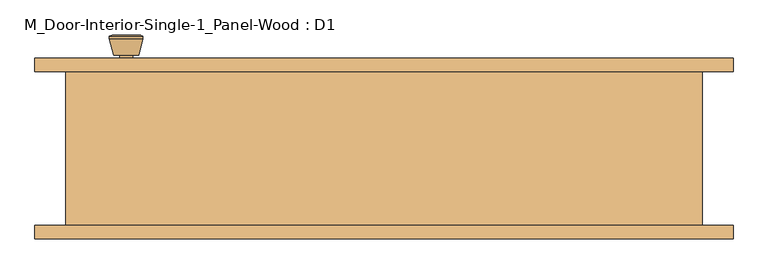
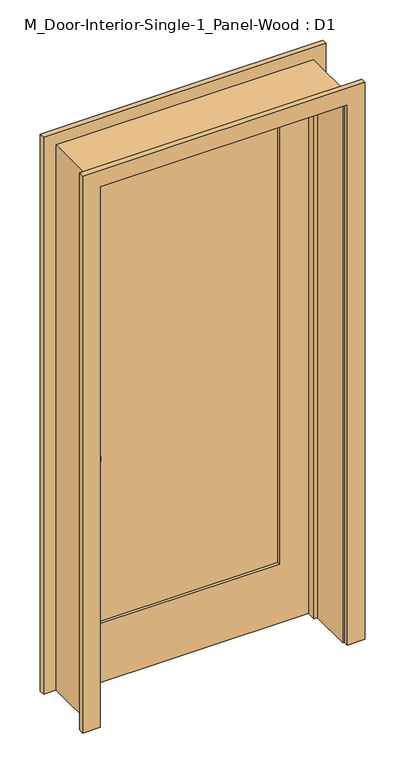
"""IFC4 building model written with IfcOpenShell, lengths in millimetres: door geometry, M_Door-Interior-Single-1_Panel-Wood : D1."""

from ifc_helpers import new_model, si_unit, point, frame, frame_2d, origin, place, context, project, spatial, polyline, circle_curve, trimmed, segment, composite_curve, outline, extrude, faceted_brep, source, transform, mapped, element, save
from ifc_brep_helpers import plane_surface, cylinder_surface, revolved_surface, advanced_brep


def m_door_interior_single_1_panel_wood_d1_706e19ec(model_context):
    return source(origin(), model_context, "Body", "SolidModel", [
        advanced_brep(
        [(-385.0, 70.825, 914.4), (-375.0, 70.825, 914.4), (-395.0, 70.825, 914.4), (-364.5241324, 21.825, 914.4), (-385.0, 21.825, 914.4), (-405.4758676, 21.825, 914.4), (-360.0, 23.6528681, 914.4), (-410.0, 23.6528681, 914.4), (-360.0, 27.1165463, 914.4), (-410.0, 27.1165463, 914.4), (-366.363764, 51.825, 914.4), (-403.636236, 51.825, 914.4), (-375.0, 51.825, 914.4), (-395.0, 51.825, 914.4)],
        [
            (0, 1),
            (1, 2, circle_curve(frame((-385.0, 70.825, 914.4), z_axis=(0.0, 1.0, 0.0), x_axis=(-1.0, 0.0, 0.0)), 10.0)),
            (2, 0),
            (2, 1, circle_curve(frame((-385.0, 70.825, 914.4), z_axis=(0.0, 1.0, 0.0), x_axis=(-1.0, 0.0, 0.0)), 10.0)),
            (3, 4),
            (4, 5),
            (5, 3, circle_curve(frame((-385.0, 21.825, 914.4), z_axis=(0.0, -1.0, 0.0), x_axis=(-1.0, 0.0, 0.0)), 20.4758676)),
            (3, 5, circle_curve(frame((-385.0, 21.825, 914.4), z_axis=(0.0, -1.0, 0.0), x_axis=(-1.0, 0.0, 0.0)), 20.4758676)),
            (6, 3),
            (5, 7),
            (7, 6, circle_curve(frame((-385.0, 23.6528681, 914.4), z_axis=(0.0, -1.0, 0.0), x_axis=(-1.0, 0.0, 0.0)), 25.0)),
            (6, 7, circle_curve(frame((-385.0, 23.6528681, 914.4), z_axis=(0.0, -1.0, 0.0), x_axis=(-1.0, 0.0, 0.0)), 25.0)),
            (8, 6),
            (7, 9),
            (9, 8, circle_curve(frame((-385.0, 27.1165463, 914.4), z_axis=(0.0, -1.0, 0.0), x_axis=(-1.0, 0.0, 0.0)), 25.0)),
            (8, 9, circle_curve(frame((-385.0, 27.1165463, 914.4), z_axis=(0.0, -1.0, 0.0), x_axis=(-1.0, 0.0, 0.0)), 25.0)),
            (10, 8),
            (9, 11),
            (11, 10, circle_curve(frame((-385.0, 51.825, 914.4), z_axis=(0.0, -1.0, 0.0), x_axis=(-1.0, 0.0, 0.0)), 18.636236)),
            (10, 11, circle_curve(frame((-385.0, 51.825, 914.4), z_axis=(0.0, -1.0, 0.0), x_axis=(-1.0, 0.0, 0.0)), 18.636236)),
            (12, 10),
            (11, 13),
            (13, 12, circle_curve(frame((-385.0, 51.825, 914.4), z_axis=(0.0, -1.0, 0.0), x_axis=(-1.0, 0.0, 0.0)), 10.0)),
            (12, 13, circle_curve(frame((-385.0, 51.825, 914.4), z_axis=(0.0, -1.0, 0.0), x_axis=(-1.0, 0.0, 0.0)), 10.0)),
            (1, 12),
            (13, 2),
        ],
        [
            plane_surface(frame((-385.0, 70.825, 914.4), z_axis=(0.0, 1.0, 0.0), x_axis=(-1.0, 0.0, 0.0))),
            plane_surface(frame((-385.0, 21.825, 914.4), z_axis=(0.0, -1.0, 0.0), x_axis=(-1.0, 0.0, 0.0))),
            revolved_surface(polyline([(-405.4758676, 21.825, 914.4), (-410.0, 23.6528681, 914.4)]), (-385.0, 70.825, 914.4), (0.0, 1.0, 0.0)),
            cylinder_surface(frame((-385.0, 70.825, 914.4), z_axis=(0.0, 1.0, 0.0), x_axis=(-1.0, 0.0, 0.0)), 25.0),
            revolved_surface(polyline([(-410.0, 27.1165463, 914.4), (-403.636236, 51.825, 914.4)]), (-385.0, 70.825, 914.4), (0.0, 1.0, 0.0)),
            plane_surface(frame((-385.0, 51.825, 914.4), z_axis=(0.0, 1.0, 0.0), x_axis=(-1.0, 0.0, 0.0))),
            cylinder_surface(frame((-385.0, 70.825, 914.4), z_axis=(0.0, 1.0, 0.0), x_axis=(-1.0, 0.0, 0.0)), 10.0),
        ],
        [
            (0, [[1, 2, 3]]),
            (0, [[-3, 4, -1]]),
            (1, [[5, 6, 7]]),
            (1, [[-6, -5, 8]]),
            (2, [[9, -7, 10, 11]]),
            (2, [[-10, -8, -9, 12]]),
            (3, [[13, -11, 14, 15]]),
            (3, [[-14, -12, -13, 16]]),
            (4, [[17, -15, 18, 19]]),
            (4, [[-18, -16, -17, 20]]),
            (5, [[21, -19, 22, 23]]),
            (5, [[-22, -20, -21, 24]]),
            (6, [[25, -23, 26, -2]]),
            (6, [[-26, -24, -25, -4]]),
        ],
    ),
        extrude(outline(composite_curve([segment(trimmed(circle_curve(frame_2d((914.4, -385.0)), 30.0), [point((914.4, -415.0))], [point((914.4, -355.0))], False, "CARTESIAN"), True, "CONTINUOUS"), segment(trimmed(circle_curve(frame_2d((914.4, -385.0)), 30.0), [point((914.4, -355.0))], [point((914.4, -415.0))], False, "CARTESIAN"), True, "CONTINUOUS")], self_intersect=False)), frame((0.0, 70.825, 0.0), z_axis=(0.0, 1.0, 0.0), x_axis=(0.0, 0.0, 1.0)), (0.0, 0.0, 1.0), 6.0),
        advanced_brep(
        [(-385.0, 117.825, 914.4), (-395.0, 117.825, 914.4), (-375.0, 117.825, 914.4), (-364.5241324, 166.825, 914.4), (-405.4758676, 166.825, 914.4), (-385.0, 166.825, 914.4), (-360.0, 164.9971319, 914.4), (-410.0, 164.9971319, 914.4), (-360.0, 161.5334537, 914.4), (-410.0, 161.5334537, 914.4), (-366.363764, 136.825, 914.4), (-403.636236, 136.825, 914.4), (-375.0, 136.825, 914.4), (-395.0, 136.825, 914.4)],
        [
            (0, 1),
            (1, 2, circle_curve(frame((-385.0, 117.825, 914.4), z_axis=(0.0, -1.0, 0.0), x_axis=(-1.0, 0.0, 0.0)), 10.0)),
            (2, 0),
            (2, 1, circle_curve(frame((-385.0, 117.825, 914.4), z_axis=(0.0, -1.0, 0.0), x_axis=(-1.0, 0.0, 0.0)), 10.0)),
            (3, 4, circle_curve(frame((-385.0, 166.825, 914.4), z_axis=(0.0, 1.0, 0.0), x_axis=(-1.0, 0.0, 0.0)), 20.4758676)),
            (4, 5),
            (5, 3),
            (4, 3, circle_curve(frame((-385.0, 166.825, 914.4), z_axis=(0.0, 1.0, 0.0), x_axis=(-1.0, 0.0, 0.0)), 20.4758676)),
            (6, 7, circle_curve(frame((-385.0, 164.9971319, 914.4), z_axis=(0.0, 1.0, 0.0), x_axis=(-1.0, 0.0, 0.0)), 25.0)),
            (7, 4),
            (3, 6),
            (7, 6, circle_curve(frame((-385.0, 164.9971319, 914.4), z_axis=(0.0, 1.0, 0.0), x_axis=(-1.0, 0.0, 0.0)), 25.0)),
            (8, 9, circle_curve(frame((-385.0, 161.5334537, 914.4), z_axis=(0.0, 1.0, 0.0), x_axis=(-1.0, 0.0, 0.0)), 25.0)),
            (9, 7),
            (6, 8),
            (9, 8, circle_curve(frame((-385.0, 161.5334537, 914.4), z_axis=(0.0, 1.0, 0.0), x_axis=(-1.0, 0.0, 0.0)), 25.0)),
            (10, 11, circle_curve(frame((-385.0, 136.825, 914.4), z_axis=(0.0, 1.0, 0.0), x_axis=(-1.0, 0.0, 0.0)), 18.636236)),
            (11, 9),
            (8, 10),
            (11, 10, circle_curve(frame((-385.0, 136.825, 914.4), z_axis=(0.0, 1.0, 0.0), x_axis=(-1.0, 0.0, 0.0)), 18.636236)),
            (12, 13, circle_curve(frame((-385.0, 136.825, 914.4), z_axis=(0.0, 1.0, 0.0), x_axis=(-1.0, 0.0, 0.0)), 10.0)),
            (13, 11),
            (10, 12),
            (13, 12, circle_curve(frame((-385.0, 136.825, 914.4), z_axis=(0.0, 1.0, 0.0), x_axis=(-1.0, 0.0, 0.0)), 10.0)),
            (1, 13),
            (12, 2),
        ],
        [
            plane_surface(frame((-385.0, 117.825, 914.4), z_axis=(0.0, -1.0, 0.0), x_axis=(-1.0, 0.0, 0.0))),
            plane_surface(frame((-385.0, 166.825, 914.4), z_axis=(0.0, 1.0, 0.0), x_axis=(-1.0, 0.0, 0.0))),
            revolved_surface(polyline([(-405.4758676, 166.825, 914.4), (-410.0, 164.9971319, 914.4)]), (-385.0, 117.825, 914.4), (0.0, -1.0, 0.0)),
            cylinder_surface(frame((-385.0, 117.825, 914.4), z_axis=(0.0, -1.0, 0.0), x_axis=(-1.0, 0.0, 0.0)), 25.0),
            revolved_surface(polyline([(-410.0, 161.5334537, 914.4), (-403.636236, 136.825, 914.4)]), (-385.0, 117.825, 914.4), (0.0, -1.0, 0.0)),
            plane_surface(frame((-385.0, 136.825, 914.4), z_axis=(0.0, -1.0, 0.0), x_axis=(-1.0, 0.0, 0.0))),
            cylinder_surface(frame((-385.0, 117.825, 914.4), z_axis=(0.0, -1.0, 0.0), x_axis=(-1.0, 0.0, 0.0)), 10.0),
        ],
        [
            (0, [[1, 2, 3]]),
            (0, [[-3, 4, -1]]),
            (1, [[5, 6, 7]]),
            (1, [[8, -7, -6]]),
            (2, [[9, 10, -5, 11]]),
            (2, [[12, -11, -8, -10]]),
            (3, [[13, 14, -9, 15]]),
            (3, [[16, -15, -12, -14]]),
            (4, [[17, 18, -13, 19]]),
            (4, [[20, -19, -16, -18]]),
            (5, [[21, 22, -17, 23]]),
            (5, [[24, -23, -20, -22]]),
            (6, [[-2, 25, -21, 26]]),
            (6, [[-4, -26, -24, -25]]),
        ],
    ),
        extrude(outline(composite_curve([segment(trimmed(circle_curve(frame_2d((914.4, -385.0)), 30.0), [point((914.4, -415.0))], [point((914.4, -355.0))], False, "CARTESIAN"), True, "CONTINUOUS"), segment(trimmed(circle_curve(frame_2d((914.4, -385.0)), 30.0), [point((914.4, -355.0))], [point((914.4, -415.0))], False, "CARTESIAN"), True, "CONTINUOUS")], self_intersect=False)), frame((0.0, 111.825, 0.0), z_axis=(0.0, 1.0, 0.0), x_axis=(0.0, 0.0, 1.0)), (0.0, 0.0, 1.0), 6.0),
        extrude(outline(polyline([(330.0, 88.4916667), (-330.0, 88.4916667), (-330.0, 100.1583333), (330.0, 100.1583333), (330.0, 88.4916667)])), frame((0.0, 0.0, 230.0), z_axis=(0.0, 0.0, 1.0), x_axis=(1.0, 0.0, 0.0)), (0.0, 0.0, 1.0), 1750.0),
        extrude(outline(polyline([(2100.0, -450.0), (0.0, -450.0), (0.0, 450.0), (2100.0, 450.0), (2100.0, -450.0)]), holes=[polyline([(1980.0, -330.0), (1980.0, 330.0), (230.0, 330.0), (230.0, -330.0), (1980.0, -330.0)])]), frame((0.0, 76.825, 0.0), z_axis=(0.0, 1.0, 0.0), x_axis=(0.0, 0.0, 1.0)), (0.0, 0.0, 1.0), 35.0),
        faceted_brep([(475.0, 111.825, 0.0), (475.0, -118.175, 0.0), (450.0, -118.175, 0.0), (450.0, 41.9, 0.0), (437.3, 41.9, 0.0), (437.3, 76.825, 0.0), (450.0, 76.825, 0.0), (450.0, 111.825, 0.0), (475.0, 111.825, 2125.0), (475.0, -118.175, 2125.0), (-475.0, -118.175, 2125.0), (-475.0, -118.175, 0.0), (-450.0, -118.175, 0.0), (-450.0, -118.175, 2100.0), (450.0, -118.175, 2100.0), (450.0, 41.9, 2100.0), (-450.0, 41.9, 2100.0), (-450.0, 41.9, 0.0), (-437.3, 41.9, 0.0), (-437.3, 41.9, 2087.3), (437.3, 41.9, 2087.3), (437.3, 76.825, 2087.3), (-437.3, 76.825, 2087.3), (-437.3, 76.825, 0.0), (-450.0, 76.825, 0.0), (-450.0, 76.825, 2100.0), (450.0, 76.825, 2100.0), (450.0, 111.825, 2100.0), (-450.0, 111.825, 2100.0), (-450.0, 111.825, 0.0), (-475.0, 111.825, 0.0), (-475.0, 111.825, 2125.0)], [[[0, 1, 2, 3, 4, 5, 6, 7]], [[1, 0, 8, 9]], [[2, 1, 9, 10, 11, 12, 13, 14]], [[3, 2, 14, 15]], [[4, 3, 15, 16, 17, 18, 19, 20]], [[5, 4, 20, 21]], [[6, 5, 21, 22, 23, 24, 25, 26]], [[7, 6, 26, 27]], [[0, 7, 27, 28, 29, 30, 31, 8]], [[9, 8, 31, 10]], [[15, 14, 13, 16]], [[21, 20, 19, 22]], [[27, 26, 25, 28]], [[30, 29, 24, 23, 18, 17, 12, 11]], [[10, 31, 30, 11]], [[16, 13, 12, 17]], [[22, 19, 18, 23]], [[28, 25, 24, 29]]]),
        extrude(outline(polyline([(0.0, 456.35), (0.0, 521.35), (2171.35, 521.35), (2171.35, -521.35), (0.0, -521.35), (0.0, -456.35), (2106.35, -456.35), (2106.35, 456.35), (0.0, 456.35)])), frame((0.0, -138.175, 0.0), z_axis=(0.0, 1.0, 0.0), x_axis=(0.0, 0.0, 1.0)), (0.0, 0.0, 1.0), 20.0),
        extrude(outline(polyline([(0.0, 456.35), (0.0, 521.35), (2171.35, 521.35), (2171.35, -521.35), (0.0, -521.35), (0.0, -456.35), (2106.35, -456.35), (2106.35, 456.35), (0.0, 456.35)])), frame((0.0, 111.825, 0.0), z_axis=(0.0, 1.0, 0.0), x_axis=(0.0, 0.0, 1.0)), (0.0, 0.0, 1.0), 20.0),
    ])


if __name__ == "__main__":
    model = new_model("IFC4")
    model_context = context("Model", 3, world=origin())
    ifc_project = project(units=[si_unit("LENGTHUNIT", "METRE", prefix="MILLI")], contexts=[model_context])
    site = spatial("IfcSite", under=ifc_project)
    building = spatial("IfcBuilding", under=site)
    placement = place(None, origin())
    m_door_interior_single_1_panel_wood_d1_shape = m_door_interior_single_1_panel_wood_d1_706e19ec(model_context)
    element("IfcDoor", 1, ObjectType="M_Door-Interior-Single-1_Panel-Wood : D1", at=placement, inside=building, context=model_context, shape_type="MappedRepresentation", body=[
        mapped(m_door_interior_single_1_panel_wood_d1_shape, transform((0.0, 0.0, 0.0), x_axis=(1.0, 0.0, 0.0), y_axis=(0.0, 1.0, 0.0), z_axis=(0.0, 0.0, 1.0))),
    ])
    save(model, "model.ifc")

# Revit data of these elements
# Type "M_Door-Interior-Single-1_Panel-Wood : D1"
#   Type Mark = "49"
#   Assembly Code = "C1020300"
#   Analytic Construction = "Wooden"
#   Top Rail = 0.12 m
#   Thickness = 0.035 m
#   Thermal Resistance (R) = 0.455703 (m²·K)/W
#   Swing Angle [instance default] = 90.00°
#   Stiles = 0.12 m
#   Rough Width = 0.95 m
#   Rough Height = 2.125 m
#   Height = 2.1 m
#   Width = 0.9 m
#   Heat Transfer Coefficient (U) = 2.19465 W/(m²·K)
#   Bottom Rail = 0.23 m
#   Trim Material = Cherry
#   Panel Material = Cherry
#   Frame Material = Cherry
#   Door Handle Material = Aluminum
#   Visual Light Transmittance = 0
#   Solar Heat Gain Coefficient = 0
#   Wall Closure = (empty or 0)
#   Function = (empty or 0)
# Element 1 (IfcDoor, "M_Door-Interior-Single-1_Panel-Wood : D1")
#   Materials on its faces: "Cherry", "Aluminum"
# Materials
#   "Cherry": class "Wood", colour RGB 226 177 128, transparency 0, Description = "Prunus Serotina", Cost = 0
#   "Aluminum": class "Metal", colour RGB 247 247 247, transparency 0, Description = "Aluminum 6061", Cost = 0
